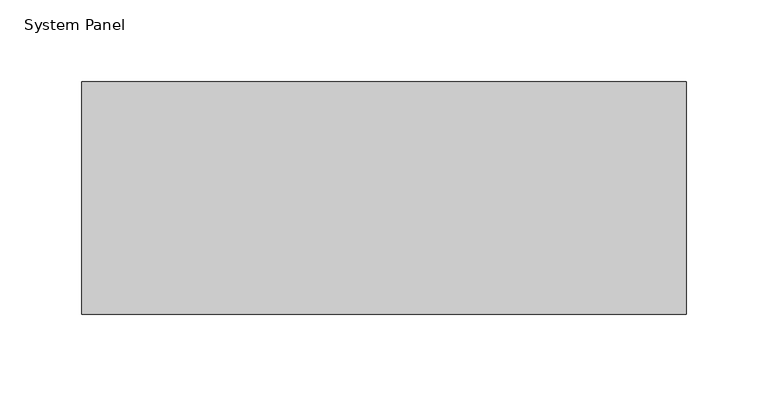
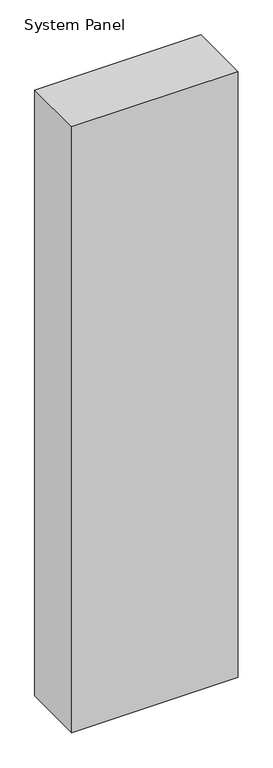
"""IFC4 building model written with IfcOpenShell, lengths in millimetres: plate geometry, System Panel : NLRS_21_CWP_hsb-vulling minerale wol 142 _gen_rsf."""

from ifc_helpers import new_model, si_unit, origin, origin_with_axes, place, context, project, spatial, polyline, outline, extrude, source, transform, mapped, element, save


def system_panel_98500bb3(model_context):
    return source(origin(), model_context, "Body", "SweptSolid", [
        extrude(outline(polyline([(184.5, -71.0), (-184.5, -71.0), (-184.5, 71.0), (184.5, 71.0), (184.5, -71.0)])), origin_with_axes(), (0.0, 0.0, 1.0), 1421.0),
    ])


if __name__ == "__main__":
    model = new_model("IFC4")
    model_context = context("Model", 3, world=origin())
    ifc_project = project(units=[si_unit("LENGTHUNIT", "METRE", prefix="MILLI")], contexts=[model_context])
    site = spatial("IfcSite", under=ifc_project)
    building = spatial("IfcBuilding", under=site)
    placement = place(None, origin())
    system_panel_shape = system_panel_98500bb3(model_context)
    element("IfcPlate", 1, ObjectType="System Panel : NLRS_21_CWP_hsb-vulling minerale wol 142 _gen_rsf", at=placement, inside=building, context=model_context, shape_type="MappedRepresentation", body=[
        mapped(system_panel_shape, transform((0.0, 0.0, 0.0), x_axis=(1.0, 0.0, 0.0), y_axis=(0.0, 1.0, 0.0), z_axis=(0.0, 0.0, 1.0))),
    ])
    save(model, "model.ifc")

# Revit data of these elements
# Type "System Panel : NLRS_21_CWP_hsb-vulling minerale wol 142 _gen_rsf"
#   Export Type to IFC As = "IfcWall"
#   Type IfcGUID = "07M7mRoiH1CR8m_RSKIwpC"
#   Assembly Code = "21.23"
# Element 1 (IfcPlate, "System Panel : NLRS_21_CWP_hsb-vulling minerale wol 142 _gen_rsf")
#   Materials on its faces: "NLRS_m1_isolatie minerale wol_gen_rsf"
# Materials
#   "NLRS_m1_isolatie minerale wol_gen_rsf": class "M - Anorganische materialen", colour RGB 200 200 140, transparency 0, Keynote = "m1", Manufacturer = "Revit Standards Foundation", URL = "www.revitstandards.org", Description = "isolatie minerale wol", Cost = 0
